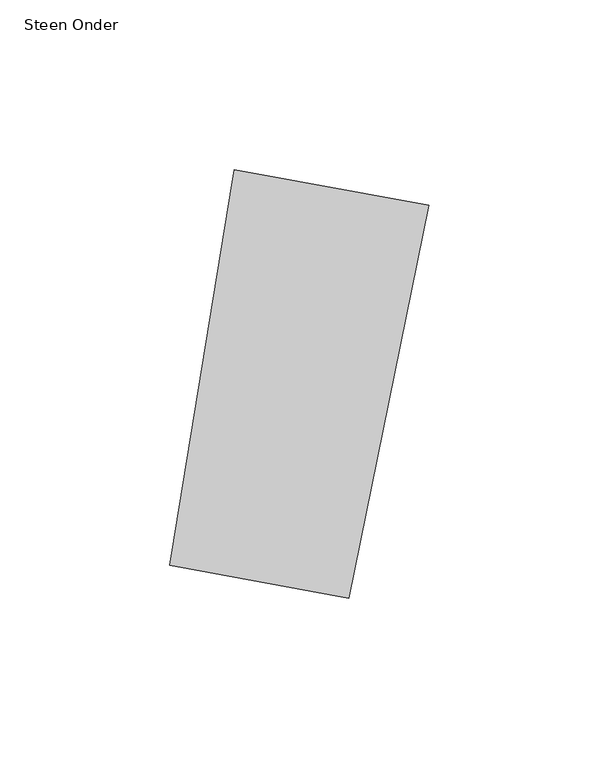
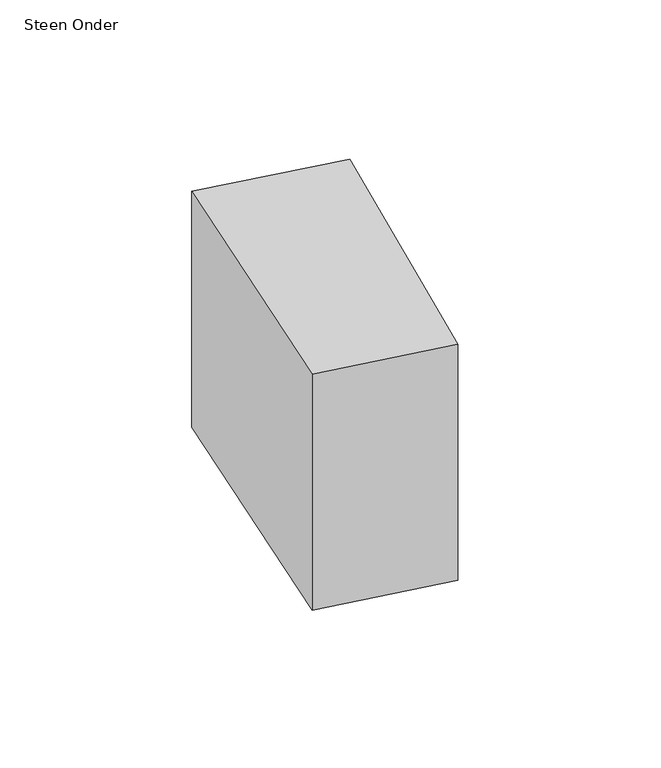
"""IFC4 building model written with IfcOpenShell, lengths in millimetres: proxy geometry, 00_GMA_steen_versie_4 : Steen Onder."""

from ifc_helpers import new_model, si_unit, origin, origin_with_axes, place, context, project, spatial, polyline, outline, extrude, source, transform, mapped, element, save


def steen_onder_4f17d981(model_context):
    return source(origin(), model_context, "Body", "SweptSolid", [
        extrude(outline(polyline([(111.9964632, 125.1842928), (88.3396843, 9.2544722), (35.4888036, 18.963932), (54.5819702, 135.7321532), (111.9964632, 125.1842928)])), origin_with_axes(), (0.0, 0.0, 1.0), 100.0),
    ])


if __name__ == "__main__":
    model = new_model("IFC4")
    model_context = context("Model", 3, world=origin())
    ifc_project = project(units=[si_unit("LENGTHUNIT", "METRE", prefix="MILLI")], contexts=[model_context])
    site = spatial("IfcSite", under=ifc_project)
    building = spatial("IfcBuilding", under=site)
    placement = place(None, origin())
    steen_onder_shape = steen_onder_4f17d981(model_context)
    element("IfcBuildingElementProxy", 1, Name="00_GMA_steen_versie_4 : Steen Onder", ObjectType="00_GMA_steen_versie_4 : Steen Onder", at=placement, inside=building, context=model_context, shape_type="MappedRepresentation", body=[
        mapped(steen_onder_shape, transform((0.0, 0.0, 0.0), x_axis=(1.0, 0.0, 0.0), y_axis=(0.0, 1.0, 0.0), z_axis=(0.0, 0.0, 1.0))),
    ])
    save(model, "model.ifc")

# Revit data of these elements
# Type "00_GMA_steen_versie_4 : Steen Onder"
#   StootVoegHalfBoven [instance default] = 5 mm
#   StootVoegHalf [instance default] = 5 mm
#   StootVoegBreedteOnder = 10 mm
#   StootVoegBreedteBoven = 10 mm
#   Steendikte = 100 mm
#   LintVoegOnderHalf = 0 mm
#   LintVoegOnder = 0 mm
#   LintVoegBovenHalf = 5 mm
#   LintVoegBoven = 10 mm
#   materiaal = none
#   MateriaalVoeg = none
#   Default Elevation = 0
